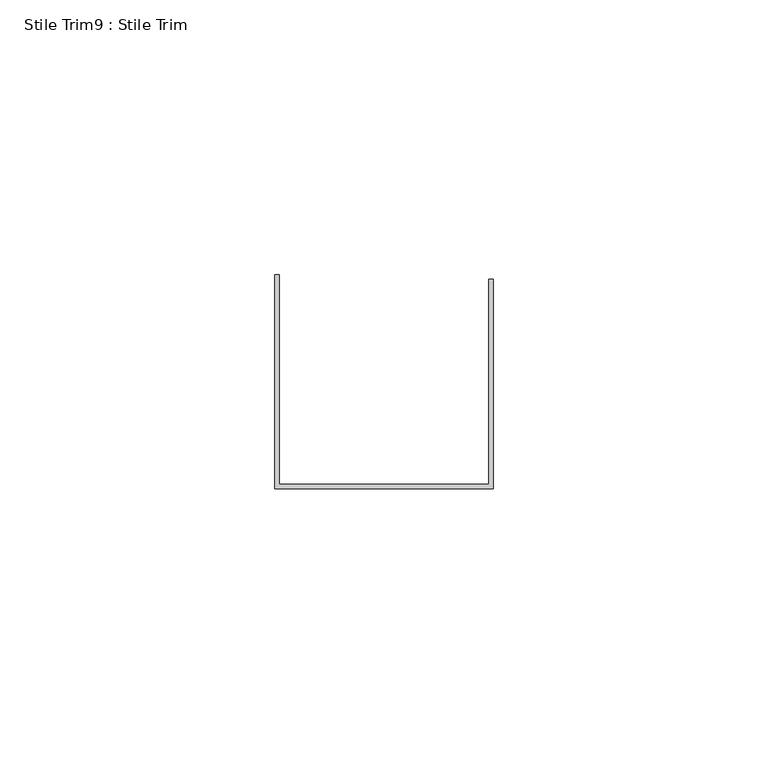
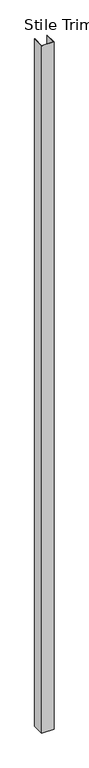
"""IFC4 building model written with IfcOpenShell, lengths in millimetres: proxy geometry, Stile Trim9 : Stile Trim."""

from ifc_helpers import new_model, si_unit, frame, origin, place, context, project, spatial, polyline, outline, extrude, source, transform, mapped, element, save


def stile_trim9_stile_trim_9ce5906b(model_context):
    return source(origin(), model_context, "Body", "SweptSolid", [
        extrude(outline(polyline([(587327.0060739, -536302.4912841), (587327.0060739, -536263.6038841), (587327.7934739, -536263.6038841), (587327.7934739, -536301.7038841), (587365.8934739, -536301.7038841), (587365.8934739, -536264.3912841), (587366.6808739, -536264.3912841), (587366.6808739, -536302.4912841), (587327.0060739, -536302.4912841)])), frame((0.0, 0.0, 50.8), z_axis=(0.0, 0.0, 1.0), x_axis=(1.0, 0.0, 0.0)), (0.0, 0.0, 1.0), 2350.3929688),
    ])


if __name__ == "__main__":
    model = new_model("IFC4")
    model_context = context("Model", 3, world=origin())
    ifc_project = project(units=[si_unit("LENGTHUNIT", "METRE", prefix="MILLI")], contexts=[model_context])
    site = spatial("IfcSite", under=ifc_project)
    building = spatial("IfcBuilding", under=site)
    placement = place(None, origin())
    stile_trim9_stile_trim_shape = stile_trim9_stile_trim_9ce5906b(model_context)
    element("IfcBuildingElementProxy", 1, Name="Stile Trim9 : Stile Trim", ObjectType="Stile Trim9 : Stile Trim", at=placement, inside=building, context=model_context, shape_type="MappedRepresentation", body=[
        mapped(stile_trim9_stile_trim_shape, transform((0.0, 0.0, 0.0), x_axis=(1.0, 0.0, 0.0), y_axis=(0.0, 1.0, 0.0), z_axis=(0.0, 0.0, 1.0))),
    ])
    save(model, "model.ifc")

# Revit data of these elements
# Element 1 (IfcBuildingElementProxy, "Stile Trim9 : Stile Trim")
#   Materials on its faces: "EDGE TRIM BY MTL PANEL MFR."
# Materials
#   "EDGE TRIM BY MTL PANEL MFR.": class "Generic", colour RGB 239 242 240, transparency 0, Cost = 0
